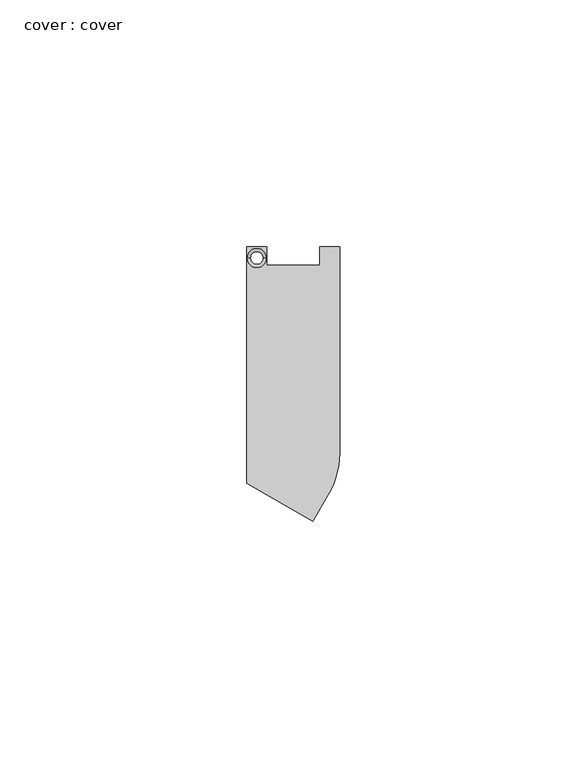
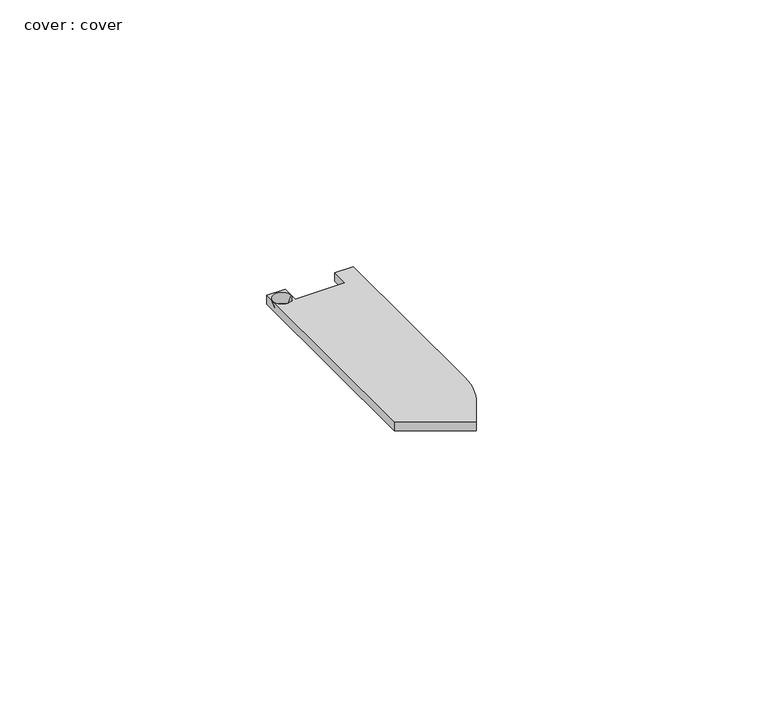
"""IFC4 building model written with IfcOpenShell, lengths in millimetres: proxy geometry, cover : cover."""

from ifc_helpers import new_model, si_unit, frame, origin, place, context, project, spatial, polyline, circle_curve, source, transform, mapped, element, save
from ifc_brep_helpers import plane_surface, revolved_surface, advanced_brep


def cover_cover_4b0dd7c3(model_context):
    return source(origin(), model_context, "Body", "AdvancedBrep", [
        advanced_brep(
        [(4663.3311724, 3530.8564939, 2.0), (4676.6686902, 3523.1530364, 2.0), (4680.3669524, 3529.5586705, 2.0), (4680.8851124, 3530.7118305, 2.0), (4681.3143724, 3531.9030905, 2.0), (4681.6547324, 3533.1222905, 2.0), (4681.9011124, 3534.3618105, 2.0), (4682.0560524, 3535.6191105, 2.0), (4682.1119324, 3536.8840305, 2.0), (4682.1119324, 3578.6670305, 2.0), (4678.1114324, 3578.6670305, 2.0), (4678.1114324, 3574.9179905, 2.0), (4667.3316724, 3574.9179905, 2.0), (4667.3314224, 3576.4165905, 2.0), (4663.3314224, 3576.4165905, 2.0), (4667.3316724, 3578.6670305, 2.0), (4663.3311724, 3578.6670305, 2.0), (4663.3311724, 3578.6670305, 0.0), (4667.3316724, 3578.6670305, 0.0), (4667.3316724, 3574.9179905, 0.0), (4678.1114324, 3574.9179905, 0.0), (4678.1114324, 3578.6670305, 0.0), (4682.1119324, 3578.6670305, 0.0), (4682.1119324, 3536.8840305, 0.0), (4682.0560524, 3535.6191105, 0.0), (4681.9011124, 3534.3618105, 0.0), (4681.6547324, 3533.1222905, 0.0), (4681.3143724, 3531.9030905, 0.0), (4680.8851124, 3530.7118305, 0.0), (4680.3669524, 3529.5586705, 0.0), (4676.6686902, 3523.1530364, 0.0), (4663.3311724, 3530.8564939, 0.0), (4664.0314224, 3576.4165905, 0.0), (4666.6314224, 3576.4165905, 0.0)],
        [
            (0, 1),
            (1, 2),
            (2, 3),
            (3, 4),
            (4, 5),
            (5, 6),
            (6, 7),
            (7, 8),
            (8, 9),
            (9, 10),
            (10, 11),
            (11, 12),
            (12, 13),
            (13, 14, circle_curve(frame((4665.3314224, 3576.4165905, 2.0), z_axis=(0.0, 0.0, -1.0), x_axis=(-1.0, 0.0, 0.0)), 2.0)),
            (14, 0),
            (15, 16),
            (16, 14),
            (14, 13, circle_curve(frame((4665.3314224, 3576.4165905, 2.0), z_axis=(0.0, 0.0, -1.0), x_axis=(1.0, 0.0, 0.0)), 2.0)),
            (13, 15),
            (17, 18),
            (18, 19),
            (19, 20),
            (20, 21),
            (21, 22),
            (22, 23),
            (23, 24),
            (24, 25),
            (25, 26),
            (26, 27),
            (27, 28),
            (28, 29),
            (29, 30),
            (30, 31),
            (31, 17),
            (32, 33, circle_curve(frame((4665.3314224, 3576.4165905, 0.0), z_axis=(0.0, 0.0, 1.0), x_axis=(-1.0, 0.0, 0.0)), 1.3)),
            (33, 32, circle_curve(frame((4665.3314224, 3576.4165905, 0.0), z_axis=(0.0, 0.0, 1.0), x_axis=(1.0, 0.0, 0.0)), 1.3)),
            (31, 0),
            (16, 17),
            (30, 1),
            (29, 2),
            (8, 23),
            (22, 9),
            (21, 10),
            (20, 11),
            (19, 12),
            (28, 3),
            (27, 4),
            (26, 5),
            (25, 6),
            (24, 7),
            (18, 15),
            (32, 14),
            (13, 33),
        ],
        [
            plane_surface(frame((4663.3311724, 3531.8548305, 2.0), z_axis=(0.0, 0.0, 1.0), x_axis=(0.0, -1.0, 0.0))),
            plane_surface(frame((4663.3311724, 3531.8548305, 0.0), z_axis=(0.0, 0.0, -1.0), x_axis=(0.0, 1.0, 0.0))),
            plane_surface(frame((4663.3311724, 3578.6670305, 2.0), z_axis=(-1.0, 0.0, 0.0), x_axis=(0.0, 0.0, -1.0))),
            plane_surface(frame((4663.3311724, 3530.8564939, 2.0), z_axis=(-0.5001479267947955, -0.8659399813629511, 0.0), x_axis=(0.0, 0.0, -1.0))),
            plane_surface(frame((4676.6686902, 3523.1530364, 2.0), z_axis=(0.8660272939548818, -0.49999672611446655, 0.0), x_axis=(0.0, 0.0, -1.0))),
            plane_surface(frame((4682.1119324, 3536.8840305, 2.0), z_axis=(1.0, 0.0, 0.0), x_axis=(0.0, 0.0, -1.0))),
            plane_surface(frame((4682.1119324, 3578.6670305, 2.0), z_axis=(0.0, 1.0, 0.0), x_axis=(0.0, 0.0, -1.0))),
            plane_surface(frame((4678.1114324, 3578.6670305, 2.0), z_axis=(-1.0, 0.0, 0.0), x_axis=(0.0, 0.0, -1.0))),
            plane_surface(frame((4678.1114324, 3574.9179905, 2.0), z_axis=(0.0, 1.0, 0.0), x_axis=(0.0, 0.0, -1.0))),
            plane_surface(frame((4680.3669524, 3529.5586705, 2.0), z_axis=(0.91214692510674, -0.40986337603928397, 0.0), x_axis=(0.0, 0.0, -1.0))),
            plane_surface(frame((4680.8851124, 3530.7118305, 2.0), z_axis=(0.9407850831608502, -0.3390035800725891, 0.0), x_axis=(0.0, 0.0, -1.0))),
            plane_surface(frame((4681.3143724, 3531.9030905, 2.0), z_axis=(0.9631721335643817, -0.26888555395379093, 0.0), x_axis=(0.0, 0.0, -1.0))),
            plane_surface(frame((4681.6547324, 3533.1222905, 2.0), z_axis=(0.9808118970912181, -0.19495646315094542, 0.0), x_axis=(0.0, 0.0, -1.0))),
            plane_surface(frame((4681.9011124, 3534.3618105, 2.0), z_axis=(0.9924922999614717, -0.12230713191465294, 0.0), x_axis=(0.0, 0.0, -1.0))),
            plane_surface(frame((4682.0560524, 3535.6191105, 2.0), z_axis=(0.9990256352193916, -0.04413366260000536, 0.0), x_axis=(0.0, 0.0, -1.0))),
            plane_surface(frame((4667.3316724, 3574.9179905, 2.0), z_axis=(1.0, 0.0, 0.0), x_axis=(0.0, 0.0, -1.0))),
            plane_surface(frame((4667.3316724, 3578.6670305, 2.0), z_axis=(0.0, 1.0, 0.0), x_axis=(0.0, 0.0, -1.0))),
            revolved_surface(polyline([(4663.3314224, 3576.4165905, 1.9999999999999996), (4664.031422401749, 3576.4165905, 0.0)]), (4665.3314224, 3576.4165905, -3.7142857), (0.0, 0.0, 1.0)),
        ],
        [
            (0, [[1, 2, 3, 4, 5, 6, 7, 8, 9, 10, 11, 12, 13, 14, 15]]),
            (0, [[16, 17, 18, 19]]),
            (1, [[20, 21, 22, 23, 24, 25, 26, 27, 28, 29, 30, 31, 32, 33, 34], [35, 36]]),
            (2, [[-34, 37, -15, -17, 38]]),
            (3, [[-1, -37, -33, 39]]),
            (4, [[-2, -39, -32, 40]]),
            (5, [[-9, 41, -25, 42]]),
            (6, [[-10, -42, -24, 43]]),
            (7, [[-11, -43, -23, 44]]),
            (8, [[-12, -44, -22, 45]]),
            (9, [[-3, -40, -31, 46]]),
            (10, [[-4, -46, -30, 47]]),
            (11, [[-5, -47, -29, 48]]),
            (12, [[-6, -48, -28, 49]]),
            (13, [[-7, -49, -27, 50]]),
            (14, [[-8, -50, -26, -41]]),
            (15, [[-21, 51, -19, -13, -45]]),
            (16, [[-16, -51, -20, -38]]),
            (17, [[52, -14, 53, -35]]),
            (17, [[-52, -36, -53, -18]]),
        ],
    ),
    ])


if __name__ == "__main__":
    model = new_model("IFC4")
    model_context = context("Model", 3, world=origin())
    ifc_project = project(units=[si_unit("LENGTHUNIT", "METRE", prefix="MILLI")], contexts=[model_context])
    site = spatial("IfcSite", under=ifc_project)
    building = spatial("IfcBuilding", under=site)
    placement = place(None, origin())
    cover_cover_shape = cover_cover_4b0dd7c3(model_context)
    element("IfcBuildingElementProxy", 1, Name="cover : cover", ObjectType="cover : cover", at=placement, inside=building, context=model_context, shape_type="MappedRepresentation", body=[
        mapped(cover_cover_shape, transform((0.0, 0.0, 0.0), x_axis=(1.0, 0.0, 0.0), y_axis=(0.0, 1.0, 0.0), z_axis=(0.0, 0.0, 1.0))),
    ])
    save(model, "model.ifc")

# Revit data of these elements
# Project information
#   Data de emissão do projeto = "Data de emissão"
#   Status do projeto = "Status do projeto"
#   Nome do cliente = "Proprietário"
#   Endereço do projeto = "Insira aqui o endereço"
#   Nome do projeto = "Nome do projeto"
#   Número do projeto = "0001"
